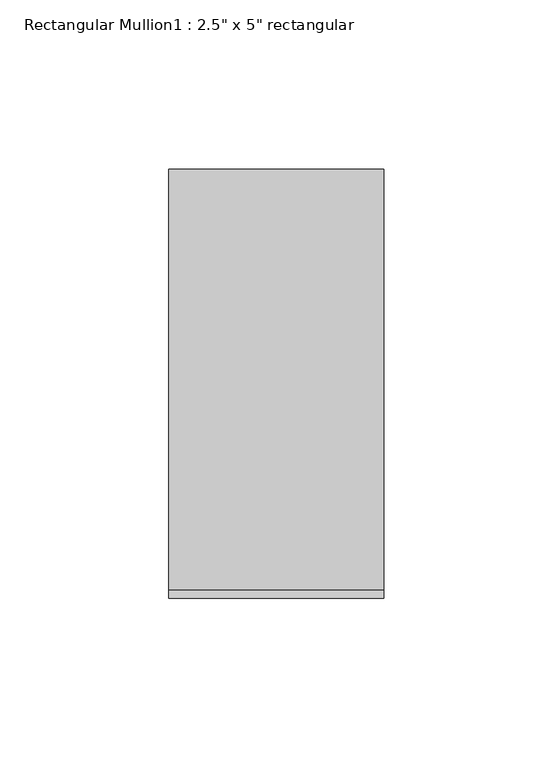
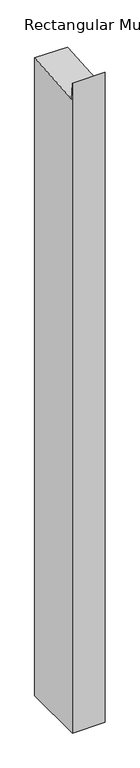
"""IFC4 building model written with IfcOpenShell, lengths in millimetres: member geometry."""

from ifc_helpers import new_model, si_unit, frame, origin, place, context, project, spatial, polyline, outline, extrude, source, transform, mapped, element, save


def member_0388ecb7(model_context):
    return source(origin(), model_context, "Body", "SweptSolid", [
        extrude(outline(polyline([(-63.5, 29.4551734), (-61.0425175, -4.5008422), (63.5, 4.512614), (63.5, -1302.7683735), (-63.5, -1302.7683735), (-63.5, 29.4551734)])), frame((-63.5, 0.0, 0.0), z_axis=(1.0, 0.0, 0.0), x_axis=(0.0, 1.0, 0.0)), (0.0, 0.0, 1.0), 63.5),
    ])


if __name__ == "__main__":
    model = new_model("IFC4")
    model_context = context("Model", 3, world=origin())
    ifc_project = project(units=[si_unit("LENGTHUNIT", "METRE", prefix="MILLI")], contexts=[model_context])
    site = spatial("IfcSite", under=ifc_project)
    building = spatial("IfcBuilding", under=site)
    placement = place(None, origin())
    member_shape = member_0388ecb7(model_context)
    element("IfcMember", 1, ObjectType="Rectangular Mullion1 : 2.5\" x 5\" rectangular", at=placement, inside=building, context=model_context, shape_type="MappedRepresentation", body=[
        mapped(member_shape, transform((0.0, 0.0, 0.0), x_axis=(1.0, 0.0, 0.0), y_axis=(0.0, 1.0, 0.0), z_axis=(0.0, 0.0, 1.0))),
    ])
    save(model, "model.ifc")

# Revit data of these elements
# Type "Rectangular Mullion1 : 2.5\" x 5\" rectangular"
#   built-in parameter 1007304 = 0.416667 (stored number, unit not read)
#   built-in parameter 1007301 = 0.104167 (stored number, unit not read)
#   built-in parameter 1007300 = 0.104167 (stored number, unit not read)
# Element 1 (IfcMember, "Rectangular Mullion1 : 2.5\" x 5\" rectangular")
#   Materials on its faces: "support-frame"
# Materials
#   "support-frame": class "Unassigned", colour RGB 233 233 233, transparency 0, Cost = 0
